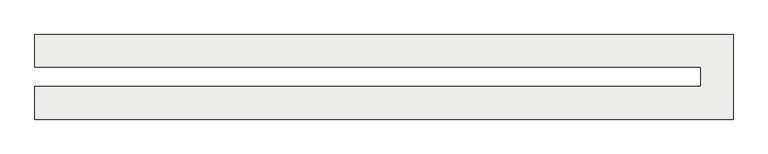
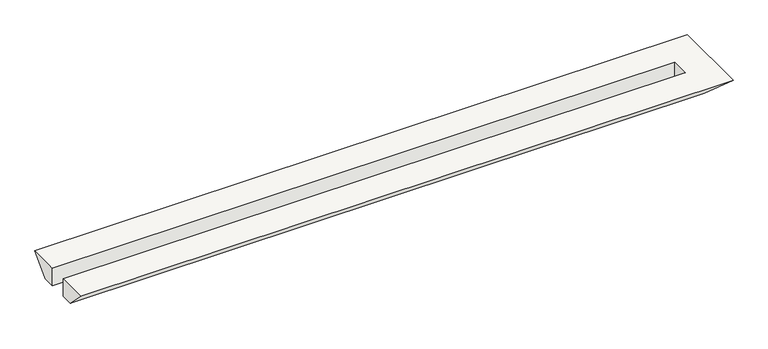
"""IFC4 building model written with IfcOpenShell, lengths in millimetres: slab geometry, Ditch Wall 1 : Ditch Wall 1."""

import ifcopenshell
import ifcopenshell.guid

model = None  # the IFC model being written
_history = None  # IfcOwnerHistory: only IFC2X3 demands one
_inside = {}  # id of a spatial element -> (the spatial element, [elements in it])
_under = {}  # id of a project, library or spatial element -> (it, [spatial elements below it])
_declared = {}  # id of a project -> (the project, [libraries it declares])
_typed = {}  # id of a type object -> (the type object, [elements of that type])
_made_of = {}  # id of a material, layer set ... -> (it, [elements and type objects made of it])


def new_model(schema):
    """Start an empty IFC model of exactly this schema.

    Asked for "IFC4X3", IfcOpenShell would pick the latest addendum, in which some entities
    have other attributes; the version numbers below select the first issue.
    IFC2X3 requires an IfcOwnerHistory on every rooted entity: one is made here for all.
    """
    global model, _history
    if schema == "IFC4X3":
        model = ifcopenshell.file(schema_version=(4, 3, 0, 0))
    else:
        model = ifcopenshell.file(schema=schema)
    _inside.clear()
    _under.clear()
    _declared.clear()
    _typed.clear()
    _made_of.clear()
    _history = None
    if model.schema == "IFC2X3":
        org = make("IfcOrganization", Name="unknown")
        user = make(
            "IfcPersonAndOrganization",
            ThePerson=make("IfcPerson", FamilyName="unknown"),
            TheOrganization=org,
        )
        app = make(
            "IfcApplication",
            ApplicationDeveloper=org,
            Version="unknown",
            ApplicationFullName="unknown",
            ApplicationIdentifier="unknown",
        )
        _history = make(
            "IfcOwnerHistory",
            OwningUser=user,
            OwningApplication=app,
            ChangeAction="ADDED",
            CreationDate=0,
        )
    return model


def make(cls, **values):
    """One entity of the class cls with the attributes given. An attribute that is None is left unset."""
    return model.create_entity(
        cls, **{name: value for name, value in values.items() if value is not None}
    )


def rooted(cls, **values):
    """An entity with a GlobalId (a new one), such as an element, a storey or a relation."""
    return make(cls, GlobalId=ifcopenshell.guid.new(), OwnerHistory=_history, **values)


def si_unit(unit_type, name, prefix=None):
    """IfcSIUnit, for example si_unit("LENGTHUNIT", "METRE", prefix="MILLI")."""
    return make("IfcSIUnit", UnitType=unit_type, Prefix=prefix, Name=name)


def assignment(units):
    """IfcUnitAssignment: the units of a project."""
    return None if units is None else make("IfcUnitAssignment", Units=units)


def point(xyz):
    """IfcCartesianPoint."""
    return None if xyz is None else make("IfcCartesianPoint", Coordinates=xyz)


def direction(xyz):
    """IfcDirection."""
    return None if xyz is None else make("IfcDirection", DirectionRatios=xyz)


def frame(location, z_axis=None, x_axis=None):
    """IfcAxis2Placement3D, a coordinate frame: its origin and axes. An axis left out is left unset."""
    return make(
        "IfcAxis2Placement3D",
        Location=point(location),
        Axis=direction(z_axis),
        RefDirection=direction(x_axis),
    )


def origin():
    """The frame at (0, 0, 0) with its axes left unset."""
    return frame((0.0, 0.0, 0.0))


def place(relative_to, where):
    """IfcLocalPlacement: puts the frame where relative to a parent placement (None: the world)."""
    return make(
        "IfcLocalPlacement", PlacementRelTo=relative_to, RelativePlacement=where
    )


def context(
    kind, dimensions, precision=None, world=None, true_north=None, identifier=None
):
    """IfcGeometricRepresentationContext, for example the 3D "Model" context."""
    return make(
        "IfcGeometricRepresentationContext",
        ContextIdentifier=identifier,
        ContextType=kind,
        CoordinateSpaceDimension=dimensions,
        Precision=precision,
        WorldCoordinateSystem=world,
        TrueNorth=true_north,
    )


def project(units=None, contexts=None):
    """IfcProject with its units and contexts."""
    return rooted(
        "IfcProject",
        Name="project",
        RepresentationContexts=contexts,
        UnitsInContext=assignment(units),
    )


def spatial(cls, under=None, at=None, **own):
    """A site, building, storey or space (cls), placed at a placement, below another one or the project."""
    s = rooted(cls, ObjectPlacement=at, **own)
    if under is not None:
        _under.setdefault(under.id(), (under, []))[1].append(s)
    return s


def faces_of(points, faces, orient=None, outer=None):
    """IfcFace entities. A face is a list of loops; a loop is a list of indices into points, from 0.

    orient and outer hold one flag for each loop. By default every Orientation is true, the
    first loop of a face is its IfcFaceOuterBound and the others are IfcFaceBound.
    """
    made = []
    for i, loops in enumerate(faces):
        bounds = []
        for j, loop in enumerate(loops):
            is_outer = j == 0 if outer is None else outer[i][j]
            bounds.append(
                make(
                    "IfcFaceOuterBound" if is_outer else "IfcFaceBound",
                    Bound=make("IfcPolyLoop", Polygon=[points[k] for k in loop]),
                    Orientation=True if orient is None else orient[i][j],
                )
            )
        made.append(make("IfcFace", Bounds=bounds))
    return made


def faceted_brep(points, faces, orient=None, outer=None, voids=None):
    """IfcFacetedBrep: a solid bounded by flat faces; with voids (closed shells), ...WithVoids."""
    shared = [point(p) for p in points]
    hull = make("IfcClosedShell", CfsFaces=faces_of(shared, faces, orient, outer))
    if voids is None:
        return make("IfcFacetedBrep", Outer=hull)
    return make(
        "IfcFacetedBrepWithVoids",
        Outer=hull,
        Voids=[
            make(cls, CfsFaces=faces_of(shared, fs, o, b)) for cls, fs, o, b in voids
        ],
    )


def shape(context_of_items, identifier, shape_type, items):
    """IfcShapeRepresentation: the items that make up one representation, for example the "Body"."""
    return make(
        "IfcShapeRepresentation",
        ContextOfItems=context_of_items,
        RepresentationIdentifier=identifier,
        RepresentationType=shape_type,
        Items=items,
    )


def source(mapping_origin, context_of_items, identifier, shape_type, items):
    """IfcRepresentationMap: a shape defined once, which mapped items show again and again."""
    return make(
        "IfcRepresentationMap",
        MappingOrigin=mapping_origin,
        MappedRepresentation=shape(context_of_items, identifier, shape_type, items),
    )


def transform(
    local_origin,
    x_axis=None,
    y_axis=None,
    z_axis=None,
    scale=None,
    scale2=None,
    scale3=None,
    uniform=True,
):
    """IfcCartesianTransformationOperator3D, or its non-uniform kind. x_axis, y_axis, z_axis: its Axis1, 2, 3."""
    if uniform:
        return make(
            "IfcCartesianTransformationOperator3D",
            Axis1=direction(x_axis),
            Axis2=direction(y_axis),
            LocalOrigin=point(local_origin),
            Scale=scale,
            Axis3=direction(z_axis),
        )
    return make(
        "IfcCartesianTransformationOperator3DnonUniform",
        Axis1=direction(x_axis),
        Axis2=direction(y_axis),
        LocalOrigin=point(local_origin),
        Scale=scale,
        Axis3=direction(z_axis),
        Scale2=scale2,
        Scale3=scale3,
    )


def mapped(mapping_source, mapping_target):
    """IfcMappedItem: shows the shape of a source again, moved by a transform."""
    return make(
        "IfcMappedItem", MappingSource=mapping_source, MappingTarget=mapping_target
    )


def made_of(thing, what):
    """Note that an element or type object is made of a material, layer set ...; save() writes the relation."""
    if what is not None:
        _made_of.setdefault(what.id(), (what, []))[1].append(thing)
    return thing


def element(
    cls,
    number,
    at=None,
    inside=None,
    cuts=None,
    type_object=None,
    material=None,
    context=None,
    identifier="Body",
    shape_type=None,
    held_by="IfcProductDefinitionShape",
    body=None,
    shapes=None,
    **own,
):
    """One element of the class cls, such as IfcWall. Its Tag is "e" and its number.

    at: its placement. inside: the storey or other place that contains it. cuts: it is an
    opening in that element (IfcRelVoidsElement). A single representation is given by context,
    identifier, shape_type and body (its items); several are given by shapes. held_by: the class
    of the entity that holds the representations. save() writes the other relations.
    """
    e = rooted(cls, Tag="e%d" % number, ObjectPlacement=at, **own)
    if body is not None:
        shapes = [shape(context, identifier, shape_type, body)]
    if shapes is not None:
        e.Representation = make(held_by, Representations=shapes)
    if inside is not None:
        _inside.setdefault(inside.id(), (inside, []))[1].append(e)
    if cuts is not None:
        rooted(
            "IfcRelVoidsElement", RelatingBuildingElement=cuts, RelatedOpeningElement=e
        )
    if type_object is not None:
        _typed.setdefault(type_object.id(), (type_object, []))[1].append(e)
    return made_of(e, material)


def aggregate(whole, parts):
    """IfcRelAggregates: a whole, such as a stair, and the parts it consists of."""
    return rooted("IfcRelAggregates", RelatingObject=whole, RelatedObjects=parts)


def save(model, path):
    """Write the relations noted so far, then the file.

    IfcRelAggregates (storeys below a building ...), IfcRelContainedInSpatialStructure (elements
    in a storey), IfcRelDefinesByType, IfcRelAssociatesMaterial and IfcRelDeclares: one each for
    every whole, place, type object, material and project.
    """
    for whole, parts in _under.values():
        aggregate(whole, parts)
    for where, things in _inside.values():
        rooted(
            "IfcRelContainedInSpatialStructure",
            RelatedElements=things,
            RelatingStructure=where,
        )
    for kind, things in _typed.values():
        rooted("IfcRelDefinesByType", RelatedObjects=things, RelatingType=kind)
    for what, things in _made_of.values():
        rooted("IfcRelAssociatesMaterial", RelatedObjects=things, RelatingMaterial=what)
    for by, libraries in _declared.values():
        rooted("IfcRelDeclares", RelatingContext=by, RelatedDefinitions=libraries)
    model.write(path)


def slab_cd841ba3(model_context):
    return source(origin(), model_context, "Body", "Brep", [
        faceted_brep([(100.0, 18494.5382614, -200.0), (100.0, 18994.5382614, -200.0), (100.0, 18694.5382614, -500.0), (100.0, 18494.5382614, -500.0), (100.0, 18494.5382614, -300.0), (10325.0, 18494.5382614, -500.0), (10325.0, 18494.5382614, -300.0), (10325.0, 18494.5382614, -200.0), (10325.0, 18194.5382614, -200.0), (100.0, 18194.5382614, -200.0), (100.0, 17694.5382614, -200.0), (10825.0, 17694.5382614, -200.0), (10825.0, 18994.5382614, -200.0), (10525.0, 18694.5382614, -500.0), (10525.0, 17994.5382614, -500.0), (100.0, 17994.5382614, -500.0), (100.0, 18194.5382614, -500.0), (10325.0, 18194.5382614, -500.0), (10325.0, 18194.5382614, -300.0), (100.0, 18194.5382614, -300.0)], [[[0, 1, 2, 3, 4]], [[3, 5, 6, 7, 0, 4]], [[1, 0, 7, 8, 9, 10, 11, 12]], [[2, 1, 12, 13]], [[3, 2, 13, 14, 15, 16, 17, 5]], [[8, 7, 6, 5, 17, 18]], [[13, 12, 11, 14]], [[10, 9, 19, 16, 15]], [[9, 8, 18, 17, 16, 19]], [[15, 14, 11, 10]]]),
    ])


if __name__ == "__main__":
    model = new_model("IFC4")
    model_context = context("Model", 3, world=origin())
    ifc_project = project(units=[si_unit("LENGTHUNIT", "METRE", prefix="MILLI")], contexts=[model_context])
    site = spatial("IfcSite", under=ifc_project)
    building = spatial("IfcBuilding", under=site)
    placement = place(None, origin())
    slab_shape = slab_cd841ba3(model_context)
    element("IfcSlab", 1, ObjectType="Ditch Wall 1 : Ditch Wall 1", at=placement, inside=building, context=model_context, shape_type="MappedRepresentation", body=[
        mapped(slab_shape, transform((0.0, 0.0, 0.0), x_axis=(1.0, 0.0, 0.0), y_axis=(0.0, 1.0, 0.0), z_axis=(0.0, 0.0, 1.0))),
    ])
    save(model, "model.ifc")

# Revit data of these elements
# Element 1 (IfcSlab, "Ditch Wall 1 : Ditch Wall 1")
#   Materials on its faces: "A03AC032-00007_Structural Concrete_Type1_25MPa-30Mpa"
# Materials
#   "A03AC032-00007_Structural Concrete_Type1_25MPa-30Mpa": class "Concrete", colour RGB 176 176 176, transparency 0, Keynote = "09910.A1", Description = "Reinf. Conc.", W00) Work Master Code = "A03AC032-00007", W01) Work Master_Lv1 = "Concrete Work", W02) Work Master_Lv2 = "Substructure Work", W03) Work Master_Spec.1 = "Structural Concrete", W04) Work Master_Spec.2 = "Cement Type-1", W05) Work Master_Spec.3 = "25MPa < F'c (Cylinder Strength) ≤ 30MPa", Cost = 0
